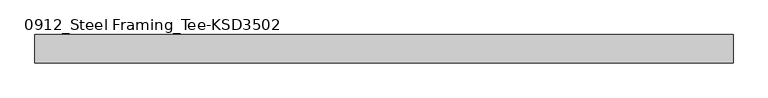
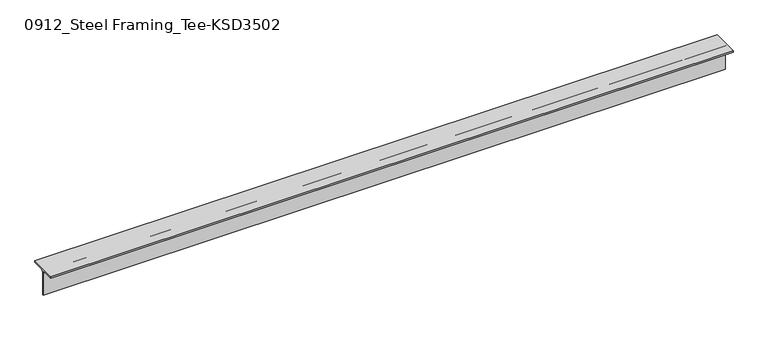
"""IFC4 building model written with IfcOpenShell, lengths in millimetres: member geometry, 0912_Steel Framing_Tee-KSD3502 : H_SB_ASB_CT-150x150x6.5x9."""

from ifc_helpers import new_model, si_unit, point, frame, frame_2d, origin, place, context, project, spatial, polyline, circle_curve, trimmed, segment, composite_curve, outline, extrude, source, transform, mapped, element, save


def member_0912_steel_framing_tee_ksd3502_3b3f0ff9(model_context):
    return source(origin(), model_context, "Body", "SweptSolid", [
        extrude(outline(composite_curve([segment(polyline([(-75.0, 75.0), (75.0, 75.0), (75.0, 66.0), (16.25, 66.0)]), True, "CONTINUOUS"), segment(trimmed(circle_curve(frame_2d((16.25, 53.0)), 13.0), [point((16.25, 66.0))], [point((3.25, 53.0))], True, "CARTESIAN"), True, "CONTINUOUS"), segment(polyline([(3.25, 53.0), (3.25, -75.0), (-3.25, -75.0), (-3.25, 53.0)]), True, "CONTINUOUS"), segment(trimmed(circle_curve(frame_2d((-16.25, 53.0)), 13.0), [point((-3.25, 53.0))], [point((-16.25, 66.0))], True, "CARTESIAN"), True, "CONTINUOUS"), segment(polyline([(-16.25, 66.0), (-75.0, 66.0), (-75.0, 75.0)]), True, "CONTINUOUS")], self_intersect=False)), frame((-1901.25, 0.0, 0.0), z_axis=(1.0, 0.0, 0.0), x_axis=(0.0, 1.0, 0.0)), (0.0, 0.0, 1.0), 3693.4),
    ])


if __name__ == "__main__":
    model = new_model("IFC4")
    model_context = context("Model", 3, world=origin())
    ifc_project = project(units=[si_unit("LENGTHUNIT", "METRE", prefix="MILLI")], contexts=[model_context])
    site = spatial("IfcSite", under=ifc_project)
    building = spatial("IfcBuilding", under=site)
    placement = place(None, origin())
    member_0912_steel_framing_tee_ksd3502_shape = member_0912_steel_framing_tee_ksd3502_3b3f0ff9(model_context)
    element("IfcMember", 1, ObjectType="0912_Steel Framing_Tee-KSD3502 : H_SB_ASB_CT-150x150x6.5x9", at=placement, inside=building, context=model_context, shape_type="MappedRepresentation", body=[
        mapped(member_0912_steel_framing_tee_ksd3502_shape, transform((0.0, 0.0, 0.0), x_axis=(1.0, 0.0, 0.0), y_axis=(0.0, 1.0, 0.0), z_axis=(0.0, 0.0, 1.0))),
    ])
    save(model, "model.ifc")

# Revit data of these elements
# Type "0912_Steel Framing_Tee-KSD3502 : H_SB_ASB_CT-150x150x6.5x9"
#   H_WM Code_1 = "S01AA003-00001 | Main Steel Structure Fabrication Work | Shelter/Building | Light Steel - Standard (30KG/M>Weight) | Material: (   )"
#   H_WM Code_2 = "S03AA029-00001 | Main Steel Structure Erection Work | Shelter/Building | Light Steel (30KG/M>Weight) | Material: (   )"
#   H_WM Code_3 = "S01AA010-00001 | Main Steel Structure Fabrication Work | Shelter/Building | Steel Painting/Coating | for Non-Fireproofed Steel Surface, Surface Preparation, Primer, Second & Final Coat | Material: (   )"
#   H_Q'ty Cal Type Tag = "SB-Q2"
#   Width = 15.0 cm
#   Web Thickness = 0.65 cm
#   Web Fillet = 1.3 cm
#   Section Area = 23.39 cm²
#   Perimeter = 0.60 m²/m
#   Nominal Weight = 18.40 kgf/m
#   Height = 15.0 cm
#   Flange Thickness = 0.9 cm
#   Centroid Vertical = 7.5 cm
#   Centroid Horizontal = 7.5 cm
#   Length [instance default] = 1.5000 m
#   Structural Material [instance default] = Steel, 45-345
#   Warping Constant = (empty or 0)
#   Torsional Moment of Inertia = 0
#   Section Name Key = ""
#   Plastic Modulus weak axis = 0
#   Plastic Modulus strong axis = 0
#   Moment of Inertia weak axis = 0
#   Moment of Inertia strong axis = 0
#   Elastic Modulus weak axis = 0
#   Elastic Modulus strong axis = 0
#   Bolt Spacing = 0
#   Assembly Code = ""
# Element 1 (IfcMember, "0912_Steel Framing_Tee-KSD3502 : H_SB_ASB_CT-150x150x6.5x9")
#   Structural Material = none
# Materials
#   "Steel, 45-345": class "Metal", colour RGB 189 187 185, transparency 0, Description = "Steel 345 MPa", Cost = 0
